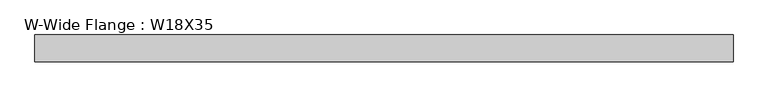
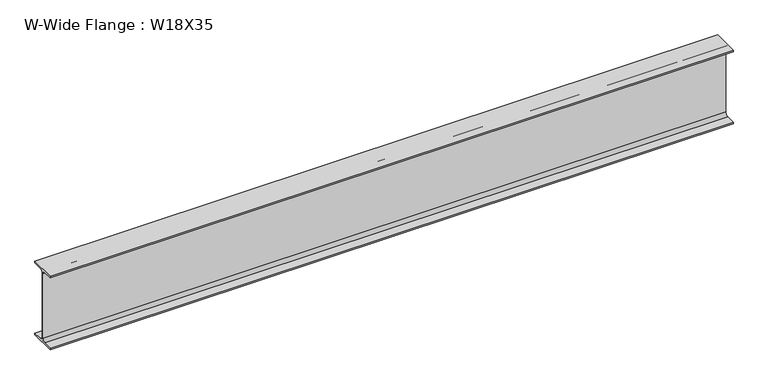
"""IFC4 building model written with IfcOpenShell, lengths in millimetres: beam geometry, W-Wide Flange : W18X35."""

from ifc_helpers import new_model, si_unit, point, frame, frame_2d, origin, place, context, project, spatial, polyline, circle_curve, trimmed, segment, composite_curve, outline, extrude, source, transform, mapped, element, save


def w_wide_flange_w18x35_d686d835(model_context):
    return source(origin(), model_context, "Body", "SweptSolid", [
        extrude(outline(composite_curve([segment(polyline([(76.2, -213.995), (76.2, -224.79), (-76.2, -224.79), (-76.2, -213.995), (-21.59, -213.995)]), True, "CONTINUOUS"), segment(trimmed(circle_curve(frame_2d((-21.59, -196.215)), 17.78), [point((-21.59, -213.995))], [point((-3.81, -196.215))], True, "CARTESIAN"), True, "CONTINUOUS"), segment(polyline([(-3.81, -196.215), (-3.81, 196.215)]), True, "CONTINUOUS"), segment(trimmed(circle_curve(frame_2d((-21.59, 196.215)), 17.78), [point((-3.81, 196.215))], [point((-21.59, 213.995))], True, "CARTESIAN"), True, "CONTINUOUS"), segment(polyline([(-21.59, 213.995), (-76.2, 213.995), (-76.2, 224.79), (76.2, 224.79), (76.2, 213.995), (21.59, 213.995)]), True, "CONTINUOUS"), segment(trimmed(circle_curve(frame_2d((21.59, 196.215)), 17.78), [point((21.59, 213.995))], [point((3.81, 196.215))], True, "CARTESIAN"), True, "CONTINUOUS"), segment(polyline([(3.81, 196.215), (3.81, -196.215)]), True, "CONTINUOUS"), segment(trimmed(circle_curve(frame_2d((21.59, -196.215)), 17.78), [point((3.81, -196.215))], [point((21.59, -213.995))], True, "CARTESIAN"), True, "CONTINUOUS"), segment(polyline([(21.59, -213.995), (76.2, -213.995)]), True, "CONTINUOUS")], self_intersect=False)), frame((-1968.5, 0.0, 0.0), z_axis=(1.0, 0.0, 0.0), x_axis=(0.0, 1.0, 0.0)), (0.0, 0.0, 1.0), 3937.0),
    ])


if __name__ == "__main__":
    model = new_model("IFC4")
    model_context = context("Model", 3, world=origin())
    ifc_project = project(units=[si_unit("LENGTHUNIT", "METRE", prefix="MILLI")], contexts=[model_context])
    site = spatial("IfcSite", under=ifc_project)
    building = spatial("IfcBuilding", under=site)
    placement = place(None, origin())
    w_wide_flange_w18x35_shape = w_wide_flange_w18x35_d686d835(model_context)
    element("IfcBeam", 1, ObjectType="W-Wide Flange : W18X35", at=placement, inside=building, context=model_context, shape_type="MappedRepresentation", body=[
        mapped(w_wide_flange_w18x35_shape, transform((0.0, 0.0, 0.0), x_axis=(1.0, 0.0, 0.0), y_axis=(0.0, 1.0, 0.0), z_axis=(0.0, 0.0, 1.0))),
    ])
    save(model, "model.ifc")

# Revit data of these elements
# Type "W-Wide Flange : W18X35"
#   Assembly Code = "B10"
#   W = 35
#   Length [instance default] = 5' - 0"
#   bf = 0' - 6"
#   d = 1' - 5.7"
#   k = 0' - 1 1/8"
#   k2 = 0' - 0.7"
#   tf = 0' - 0.425"
#   tw = 0' - 0.3"
#   A = 0.0715278 SF
#   Structural Material [instance default] = Steel ASTM A992
# Element 1 (IfcBeam, "W-Wide Flange : W18X35")
#   Structural Material = Steel ASTM A36
#   Materials on its faces: "Steel ASTM A36"
# Materials
#   "Steel ASTM A992": class "Metal", colour RGB 199 199 199, transparency 0, Description = "Structural steel 50ksi", Cost = 0
#   "Steel ASTM A36": class "Metal", colour RGB 199 199 199, transparency 0, Description = "Structural steel, ASTM A36 Grade B, mill finish", Cost = 0
